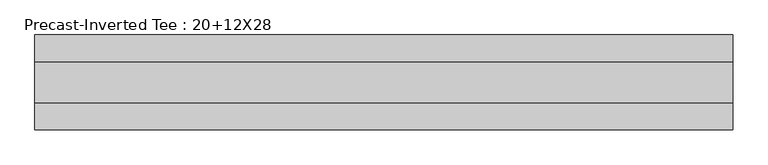
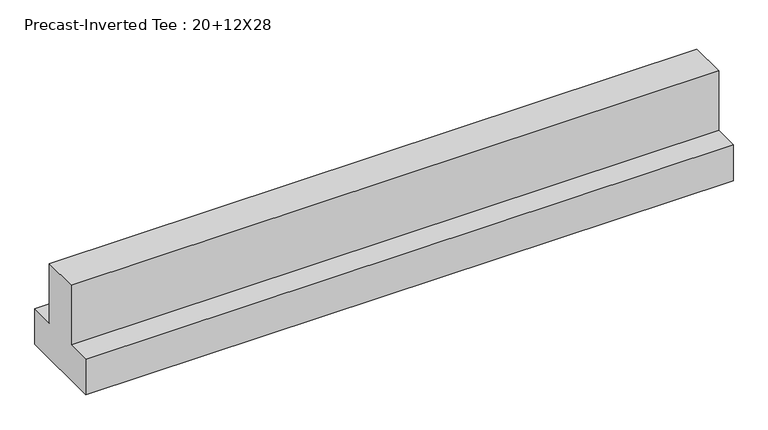
"""IFC4 building model written with IfcOpenShell, lengths in millimetres: beam geometry, Precast-Inverted Tee : 20+12X28."""

from ifc_helpers import new_model, si_unit, frame, origin, place, context, project, spatial, polyline, outline, extrude, source, transform, mapped, element, save


def precast_inverted_tee_20_12x28_b7649b98(model_context):
    return source(origin(), model_context, "Body", "SweptSolid", [
        extrude(outline(polyline([(355.6, -406.4), (-355.6, -406.4), (-355.6, -101.6), (-152.4, -101.6), (-152.4, 406.4), (152.4, 406.4), (152.4, -101.6), (355.6, -101.6), (355.6, -406.4)])), frame((-2730.5, 0.0, 0.0), z_axis=(1.0, 0.0, 0.0), x_axis=(0.0, 1.0, 0.0)), (0.0, 0.0, 1.0), 5232.4),
    ])


if __name__ == "__main__":
    model = new_model("IFC4")
    model_context = context("Model", 3, world=origin())
    ifc_project = project(units=[si_unit("LENGTHUNIT", "METRE", prefix="MILLI")], contexts=[model_context])
    site = spatial("IfcSite", under=ifc_project)
    building = spatial("IfcBuilding", under=site)
    placement = place(None, origin())
    precast_inverted_tee_20_12x28_shape = precast_inverted_tee_20_12x28_b7649b98(model_context)
    element("IfcBeam", 1, ObjectType="Precast-Inverted Tee : 20+12X28", at=placement, inside=building, context=model_context, shape_type="MappedRepresentation", body=[
        mapped(precast_inverted_tee_20_12x28_shape, transform((0.0, 0.0, 0.0), x_axis=(1.0, 0.0, 0.0), y_axis=(0.0, 1.0, 0.0), z_axis=(0.0, 0.0, 1.0))),
    ])
    save(model, "model.ifc")

# Revit data of these elements
# Type "Precast-Inverted Tee : 20+12X28"
#   Assembly Code = "B10"
#   Seat = 0' - 8"
#   Length [instance default] = 5' - 0"
#   b = 2' - 4"
#   h = 2' - 8"
#   h1 = 1' - 8"
#   Structural Material [instance default] = Concrete - Precast Concrete - Normal Weight Concrete - 5 ksi
# Element 1 (IfcBeam, "Precast-Inverted Tee : 20+12X28")
#   Length = 17' - 6"
#   Materials on its faces: "Concrete - Precast Concrete - Normal Weight Concrete - 5 ksi"
# Materials
#   "Concrete - Precast Concrete - Normal Weight Concrete - 5 ksi": class "Concrete", colour RGB 198 187 187, transparency 0, Cost = 0
